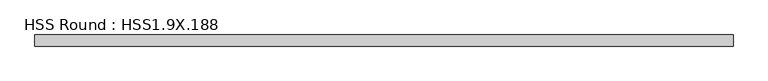
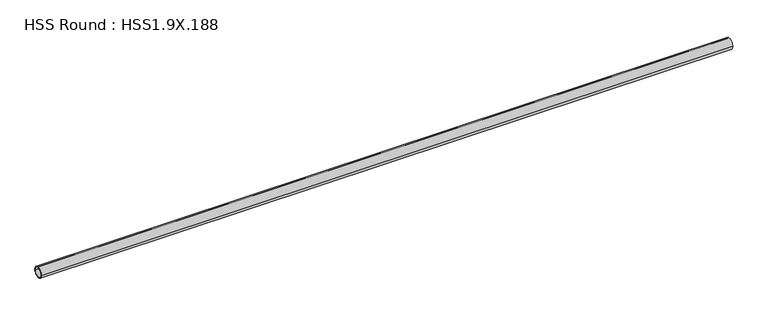
"""IFC4 building model written with IfcOpenShell, lengths in millimetres: member geometry, HSS Round : HSS1.9X.188."""

from ifc_helpers import new_model, si_unit, point, frame, origin, origin_2d, place, context, project, spatial, circle_curve, trimmed, segment, composite_curve, outline, extrude, source, transform, mapped, element, save


def hss_round_hss1_9x_188_f1efcc2e(model_context):
    return source(origin(), model_context, "Body", "SweptSolid", [
        extrude(outline(composite_curve([segment(trimmed(circle_curve(origin_2d(), 24.13), [point((-24.13, 0.0))], [point((24.13, 0.0))], False, "CARTESIAN"), True, "CONTINUOUS"), segment(trimmed(circle_curve(origin_2d(), 24.13), [point((24.13, 0.0))], [point((-24.13, 0.0))], False, "CARTESIAN"), True, "CONTINUOUS")], self_intersect=False), holes=[composite_curve([segment(trimmed(circle_curve(origin_2d(), 19.3548), [point((19.3548, 0.0))], [point((-19.3548, 0.0))], True, "CARTESIAN"), True, "CONTINUOUS"), segment(trimmed(circle_curve(origin_2d(), 19.3548), [point((-19.3548, 0.0))], [point((19.3548, 0.0))], True, "CARTESIAN"), True, "CONTINUOUS")], self_intersect=False)]), frame((-1547.6482393, 0.0, 0.0), z_axis=(1.0, 0.0, 0.0), x_axis=(0.0, 1.0, 0.0)), (0.0, 0.0, 1.0), 3024.8924552),
    ])


if __name__ == "__main__":
    model = new_model("IFC4")
    model_context = context("Model", 3, world=origin())
    ifc_project = project(units=[si_unit("LENGTHUNIT", "METRE", prefix="MILLI")], contexts=[model_context])
    site = spatial("IfcSite", under=ifc_project)
    building = spatial("IfcBuilding", under=site)
    placement = place(None, origin())
    hss_round_hss1_9x_188_shape = hss_round_hss1_9x_188_f1efcc2e(model_context)
    element("IfcMember", 1, ObjectType="HSS Round : HSS1.9X.188", at=placement, inside=building, context=model_context, shape_type="MappedRepresentation", body=[
        mapped(hss_round_hss1_9x_188_shape, transform((0.0, 0.0, 0.0), x_axis=(1.0, 0.0, 0.0), y_axis=(0.0, 1.0, 0.0), z_axis=(0.0, 0.0, 1.0))),
    ])
    save(model, "model.ifc")

# Revit data of these elements
# Type "HSS Round : HSS1.9X.188"
#   Section Name Key = "HSSRound 1.900x0.188"
#   Assembly Code = "B10"
#   Wall Nominal Thickness = 0.188"
#   Wall Design Thickness = 0.174"
#   Torsional Moment of Inertia = 0.71 in⁴
#   Torsional Modulus = 0.747 in³
#   Section Area = 0.943 in²
#   Plastic Modulus weak axis = 0.52 in³
#   Plastic Modulus strong axis = 0.52 in³
#   Nominal Weight = 3.44 lbf/ft
#   Moment of Inertia weak axis = 0.355 in⁴
#   Moment of Inertia strong axis = 0.355 in⁴
#   Elastic Modulus weak axis = 0.374 in³
#   Elastic Modulus strong axis = 0.374 in³
#   Diameter = 1.900"
#   Centroid Vertical = 0.950"
#   Centroid Horizontal = 0.950"
#   Length [instance default] = 5' - 0"
#   Structural Material [instance default] = Steel ASTM A500, Grade B, Round
#   Warping Constant = (empty or 0)
#   Principal Axes Angle = 0
# Element 1 (IfcMember, "HSS Round : HSS1.9X.188")
#   Structural Material = Steel ASTM A992
#   Materials on its faces: "Steel ASTM A992"
# Materials
#   "Steel ASTM A500, Grade B, Round": class "Metal", colour RGB 199 199 199, transparency 0, Description = "Carbon steel", Cost = 0
#   "Steel ASTM A992": class "Metal", colour RGB 199 199 199, transparency 0, Description = "Structural steel 50ksi", Cost = 0
